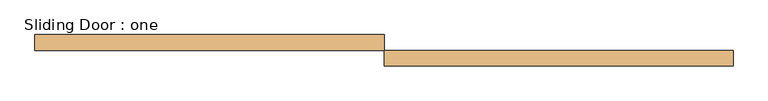
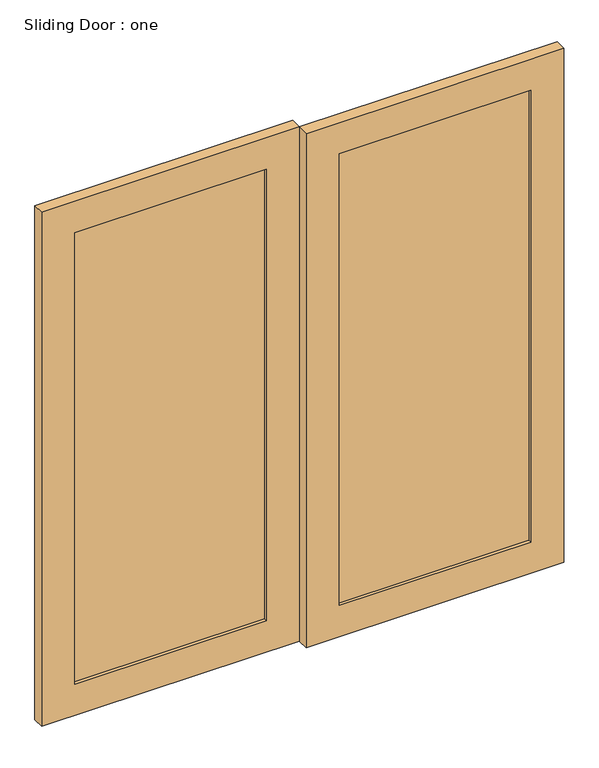
"""IFC4 building model written with IfcOpenShell, lengths in millimetres: door geometry, Sliding Door : one."""

from ifc_helpers import new_model, si_unit, frame, origin, place, context, project, spatial, polyline, outline, extrude, source, transform, mapped, element, save


def sliding_door_one_759039ca(model_context):
    return source(origin(), model_context, "Body", "SweptSolid", [
        extrude(outline(polyline([(-127.0, 50.8), (-127.0, 31.75), (-863.6, 31.75), (-863.6, 50.8), (-127.0, 50.8)])), frame((0.0, 0.0, 127.0), z_axis=(0.0, 0.0, 1.0), x_axis=(1.0, 0.0, 0.0)), (0.0, 0.0, 1.0), 1834.35625),
        extrude(outline(polyline([(863.6, 6.35), (863.6, -12.7), (127.0, -12.7), (127.0, 6.35), (863.6, 6.35)])), frame((0.0, 0.0, 127.0), z_axis=(0.0, 0.0, 1.0), x_axis=(1.0, 0.0, 0.0)), (0.0, 0.0, 1.0), 1834.35625),
        extrude(outline(polyline([(2088.35625, -990.6), (0.0, -990.6), (0.0, 0.0), (2088.35625, 0.0), (2088.35625, -990.6)]), holes=[polyline([(127.0, -127.0), (127.0, -863.6), (1961.35625, -863.6), (1961.35625, -127.0), (127.0, -127.0)])]), frame((0.0, 19.05, 0.0), z_axis=(0.0, 1.0, 0.0), x_axis=(0.0, 0.0, 1.0)), (0.0, 0.0, 1.0), 44.45),
        extrude(outline(polyline([(2088.35625, 0.0), (0.0, 0.0), (0.0, 990.6), (2088.35625, 990.6), (2088.35625, 0.0)]), holes=[polyline([(127.0, 863.6), (127.0, 127.0), (1961.35625, 127.0), (1961.35625, 863.6), (127.0, 863.6)])]), frame((0.0, -25.4, 0.0), z_axis=(0.0, 1.0, 0.0), x_axis=(0.0, 0.0, 1.0)), (0.0, 0.0, 1.0), 44.45),
    ])


if __name__ == "__main__":
    model = new_model("IFC4")
    model_context = context("Model", 3, world=origin())
    ifc_project = project(units=[si_unit("LENGTHUNIT", "METRE", prefix="MILLI")], contexts=[model_context])
    site = spatial("IfcSite", under=ifc_project)
    building = spatial("IfcBuilding", under=site)
    placement = place(None, origin())
    sliding_door_one_shape = sliding_door_one_759039ca(model_context)
    element("IfcDoor", 1, ObjectType="Sliding Door : one", at=placement, inside=building, context=model_context, shape_type="MappedRepresentation", body=[
        mapped(sliding_door_one_shape, transform((0.0, 0.0, 0.0), x_axis=(1.0, 0.0, 0.0), y_axis=(0.0, 1.0, 0.0), z_axis=(0.0, 0.0, 1.0))),
    ])
    save(model, "model.ifc")

# Revit data of these elements
# Type "Sliding Door : one"
#   Type Mark = "70"
#   OD_DS_Door_Material = "ALUM./GLAZING"
#   OD_DS_Door_Type = "STOREFRONT - SLIDING DOOR"
#   OD_DS_Lockset = "MANUAL OPENING"
#   Analytic Construction = "<None>"
#   Stile_Width = 0' - 5"
#   Door_Thickness = 0' - 1 3/4"
#   Door_Offset = 0' - 1"
#   Glass_Material = SAFETY GLAZING
#   Frame_Material = INTERIOR GRADE ALUMINUM STOREFRONT W/ SAFETY GLAZING
#   Function = (empty or 0)
# Element 1 (IfcDoor, "Sliding Door : one")
#   Materials on its faces: "INTERIOR GRADE ALUMINUM STOREFRONT W/ SAFETY GLAZING", "SAFETY GLAZING"
# Materials
#   "SAFETY GLAZING": class "Glass", colour RGB 142 168 196, transparency 0.75, Description = "Soda Lime Glass", Cost = 0
#   "INTERIOR GRADE ALUMINUM STOREFRONT W/ SAFETY GLAZING": class "Metal", colour RGB 226 226 226, transparency 0, Description = "Aluminum 6061", Cost = 0
